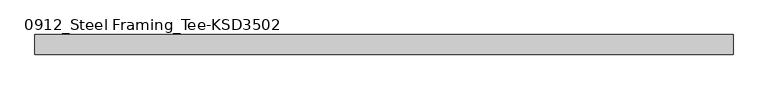
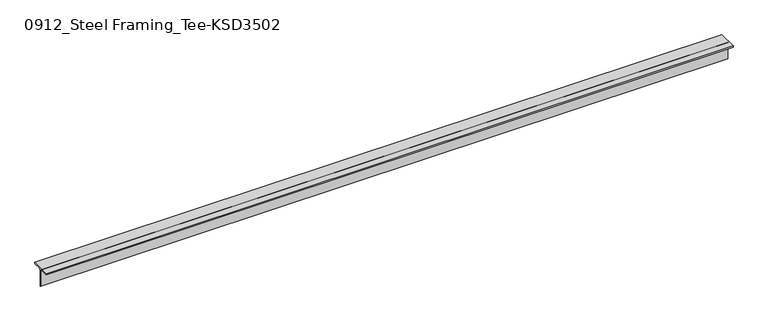
"""IFC4 building model written with IfcOpenShell, lengths in millimetres: member geometry, 0912_Steel Framing_Tee-KSD3502 : H_SB_ASB_CT-150x150x6.5x9."""

from ifc_helpers import new_model, si_unit, point, frame, frame_2d, origin, place, context, project, spatial, polyline, circle_curve, trimmed, segment, composite_curve, outline, extrude, source, transform, mapped, element, save


def member_0912_steel_framing_tee_ksd3502_b77b4f79(model_context):
    return source(origin(), model_context, "Body", "SweptSolid", [
        extrude(outline(composite_curve([segment(polyline([(-75.0, 75.0), (75.0, 75.0), (75.0, 66.0), (16.25, 66.0)]), True, "CONTINUOUS"), segment(trimmed(circle_curve(frame_2d((16.25, 53.0)), 13.0), [point((16.25, 66.0))], [point((3.25, 53.0))], True, "CARTESIAN"), True, "CONTINUOUS"), segment(polyline([(3.25, 53.0), (3.25, -75.0), (-3.25, -75.0), (-3.25, 53.0)]), True, "CONTINUOUS"), segment(trimmed(circle_curve(frame_2d((-16.25, 53.0)), 13.0), [point((-3.25, 53.0))], [point((-16.25, 66.0))], True, "CARTESIAN"), True, "CONTINUOUS"), segment(polyline([(-16.25, 66.0), (-75.0, 66.0), (-75.0, 75.0)]), True, "CONTINUOUS")], self_intersect=False)), frame((-2752.4, 0.0, 0.0), z_axis=(1.0, 0.0, 0.0), x_axis=(0.0, 1.0, 0.0)), (0.0, 0.0, 1.0), 5329.7),
    ])


if __name__ == "__main__":
    model = new_model("IFC4")
    model_context = context("Model", 3, world=origin())
    ifc_project = project(units=[si_unit("LENGTHUNIT", "METRE", prefix="MILLI")], contexts=[model_context])
    site = spatial("IfcSite", under=ifc_project)
    building = spatial("IfcBuilding", under=site)
    placement = place(None, origin())
    member_0912_steel_framing_tee_ksd3502_shape = member_0912_steel_framing_tee_ksd3502_b77b4f79(model_context)
    element("IfcMember", 1, ObjectType="0912_Steel Framing_Tee-KSD3502 : H_SB_ASB_CT-150x150x6.5x9", at=placement, inside=building, context=model_context, shape_type="MappedRepresentation", body=[
        mapped(member_0912_steel_framing_tee_ksd3502_shape, transform((0.0, 0.0, 0.0), x_axis=(1.0, 0.0, 0.0), y_axis=(0.0, 1.0, 0.0), z_axis=(0.0, 0.0, 1.0))),
    ])
    save(model, "model.ifc")

# Revit data of these elements
# Type "0912_Steel Framing_Tee-KSD3502 : H_SB_ASB_CT-150x150x6.5x9"
#   H_WM Code_1 = "S01AA003-00001 | Main Steel Structure Fabrication Work | Shelter/Building | Light Steel - Standard (30KG/M>Weight) | Material: (   )"
#   H_WM Code_2 = "S03AA029-00001 | Main Steel Structure Erection Work | Shelter/Building | Light Steel (30KG/M>Weight) | Material: (   )"
#   H_WM Code_3 = "S01AA010-00001 | Main Steel Structure Fabrication Work | Shelter/Building | Steel Painting/Coating | for Non-Fireproofed Steel Surface, Surface Preparation, Primer, Second & Final Coat | Material: (   )"
#   H_Q'ty Cal Type Tag = "SB-Q2"
#   Width = 15.0 cm
#   Web Thickness = 0.65 cm
#   Web Fillet = 1.3 cm
#   Section Area = 23.39 cm²
#   Perimeter = 0.60 m²/m
#   Nominal Weight = 18.40 kgf/m
#   Height = 15.0 cm
#   Flange Thickness = 0.9 cm
#   Centroid Vertical = 7.5 cm
#   Centroid Horizontal = 7.5 cm
#   Length [instance default] = 1.5000 m
#   Structural Material [instance default] = Steel, 45-345
#   Warping Constant = (empty or 0)
#   Torsional Moment of Inertia = 0
#   Section Name Key = ""
#   Plastic Modulus weak axis = 0
#   Plastic Modulus strong axis = 0
#   Moment of Inertia weak axis = 0
#   Moment of Inertia strong axis = 0
#   Elastic Modulus weak axis = 0
#   Elastic Modulus strong axis = 0
#   Bolt Spacing = 0
#   Assembly Code = ""
# Element 1 (IfcMember, "0912_Steel Framing_Tee-KSD3502 : H_SB_ASB_CT-150x150x6.5x9")
#   Structural Material = none
# Materials
#   "Steel, 45-345": class "Metal", colour RGB 189 187 185, transparency 0, Description = "Steel 345 MPa", Cost = 0
